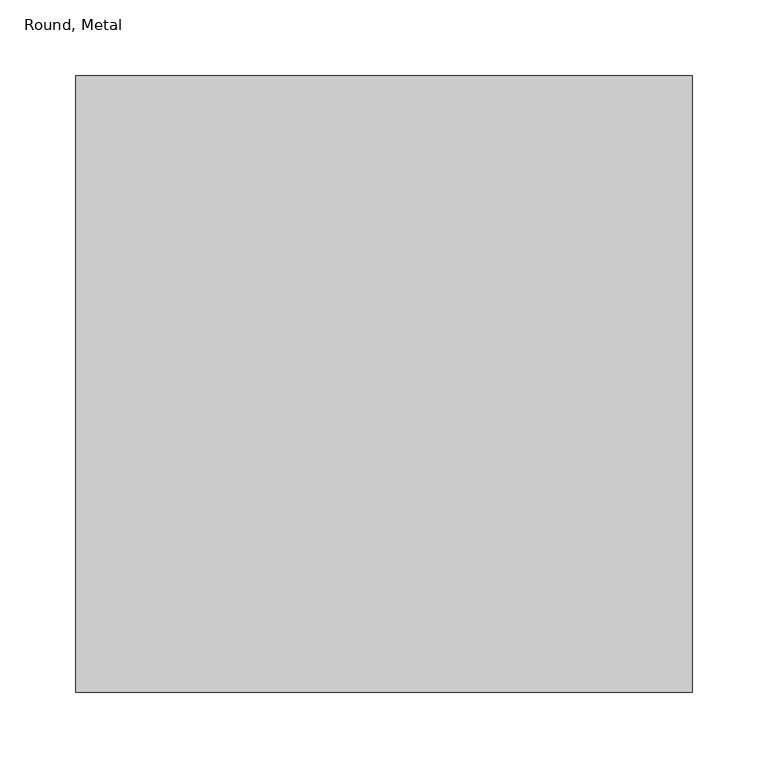
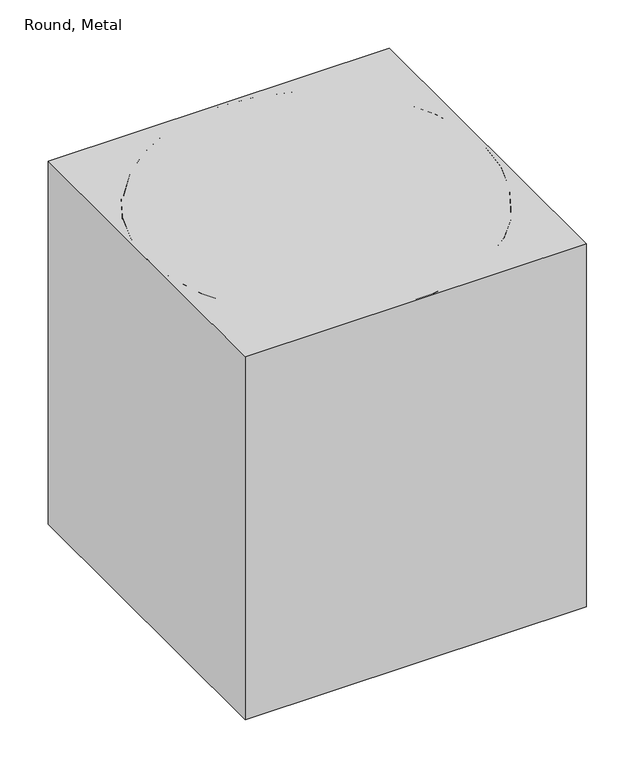
"""IFC4 building model written with IfcOpenShell, lengths in millimetres: proxy geometry, F2000 - Basket, Wastepaper : Round, Metal."""

import ifcopenshell
import ifcopenshell.guid

model = None  # the IFC model being written
_history = None  # IfcOwnerHistory: only IFC2X3 demands one
_inside = {}  # id of a spatial element -> (the spatial element, [elements in it])
_under = {}  # id of a project, library or spatial element -> (it, [spatial elements below it])
_declared = {}  # id of a project -> (the project, [libraries it declares])
_typed = {}  # id of a type object -> (the type object, [elements of that type])
_made_of = {}  # id of a material, layer set ... -> (it, [elements and type objects made of it])


def new_model(schema):
    """Start an empty IFC model of exactly this schema.

    Asked for "IFC4X3", IfcOpenShell would pick the latest addendum, in which some entities
    have other attributes; the version numbers below select the first issue.
    IFC2X3 requires an IfcOwnerHistory on every rooted entity: one is made here for all.
    """
    global model, _history
    if schema == "IFC4X3":
        model = ifcopenshell.file(schema_version=(4, 3, 0, 0))
    else:
        model = ifcopenshell.file(schema=schema)
    _inside.clear()
    _under.clear()
    _declared.clear()
    _typed.clear()
    _made_of.clear()
    _history = None
    if model.schema == "IFC2X3":
        org = make("IfcOrganization", Name="unknown")
        user = make(
            "IfcPersonAndOrganization",
            ThePerson=make("IfcPerson", FamilyName="unknown"),
            TheOrganization=org,
        )
        app = make(
            "IfcApplication",
            ApplicationDeveloper=org,
            Version="unknown",
            ApplicationFullName="unknown",
            ApplicationIdentifier="unknown",
        )
        _history = make(
            "IfcOwnerHistory",
            OwningUser=user,
            OwningApplication=app,
            ChangeAction="ADDED",
            CreationDate=0,
        )
    return model


def make(cls, **values):
    """One entity of the class cls with the attributes given. An attribute that is None is left unset."""
    return model.create_entity(
        cls, **{name: value for name, value in values.items() if value is not None}
    )


def rooted(cls, **values):
    """An entity with a GlobalId (a new one), such as an element, a storey or a relation."""
    return make(cls, GlobalId=ifcopenshell.guid.new(), OwnerHistory=_history, **values)


def si_unit(unit_type, name, prefix=None):
    """IfcSIUnit, for example si_unit("LENGTHUNIT", "METRE", prefix="MILLI")."""
    return make("IfcSIUnit", UnitType=unit_type, Prefix=prefix, Name=name)


def assignment(units):
    """IfcUnitAssignment: the units of a project."""
    return None if units is None else make("IfcUnitAssignment", Units=units)


def point(xyz):
    """IfcCartesianPoint."""
    return None if xyz is None else make("IfcCartesianPoint", Coordinates=xyz)


def direction(xyz):
    """IfcDirection."""
    return None if xyz is None else make("IfcDirection", DirectionRatios=xyz)


def frame(location, z_axis=None, x_axis=None):
    """IfcAxis2Placement3D, a coordinate frame: its origin and axes. An axis left out is left unset."""
    return make(
        "IfcAxis2Placement3D",
        Location=point(location),
        Axis=direction(z_axis),
        RefDirection=direction(x_axis),
    )


def frame_2d(location, x_axis=None):
    """IfcAxis2Placement2D, a coordinate frame in the plane: its origin and x axis."""
    return make(
        "IfcAxis2Placement2D", Location=point(location), RefDirection=direction(x_axis)
    )


def origin():
    """The frame at (0, 0, 0) with its axes left unset."""
    return frame((0.0, 0.0, 0.0))


def origin_with_axes():
    """The frame at (0, 0, 0) with the z axis (0, 0, 1) and the x axis (1, 0, 0) written out."""
    return frame((0.0, 0.0, 0.0), z_axis=(0.0, 0.0, 1.0), x_axis=(1.0, 0.0, 0.0))


def origin_2d():
    """The frame at (0, 0) in the plane with its x axis left unset."""
    return frame_2d((0.0, 0.0))


def place(relative_to, where):
    """IfcLocalPlacement: puts the frame where relative to a parent placement (None: the world)."""
    return make(
        "IfcLocalPlacement", PlacementRelTo=relative_to, RelativePlacement=where
    )


def context(
    kind, dimensions, precision=None, world=None, true_north=None, identifier=None
):
    """IfcGeometricRepresentationContext, for example the 3D "Model" context."""
    return make(
        "IfcGeometricRepresentationContext",
        ContextIdentifier=identifier,
        ContextType=kind,
        CoordinateSpaceDimension=dimensions,
        Precision=precision,
        WorldCoordinateSystem=world,
        TrueNorth=true_north,
    )


def project(units=None, contexts=None):
    """IfcProject with its units and contexts."""
    return rooted(
        "IfcProject",
        Name="project",
        RepresentationContexts=contexts,
        UnitsInContext=assignment(units),
    )


def spatial(cls, under=None, at=None, **own):
    """A site, building, storey or space (cls), placed at a placement, below another one or the project."""
    s = rooted(cls, ObjectPlacement=at, **own)
    if under is not None:
        _under.setdefault(under.id(), (under, []))[1].append(s)
    return s


def polyline(points):
    """IfcPolyline through the points."""
    return make("IfcPolyline", Points=[point(p) for p in points])


def circle_curve(where, radius):
    """IfcCircle in the frame where."""
    return make("IfcCircle", Position=where, Radius=radius)


def trimmed(basis, trim1, trim2, sense, master):
    """IfcTrimmedCurve: the piece of a basis curve between two trims."""
    return make(
        "IfcTrimmedCurve",
        BasisCurve=basis,
        Trim1=trim1,
        Trim2=trim2,
        SenseAgreement=sense,
        MasterRepresentation=master,
    )


def segment(curve, same_sense, transition):
    """IfcCompositeCurveSegment."""
    return make(
        "IfcCompositeCurveSegment",
        Transition=transition,
        SameSense=same_sense,
        ParentCurve=curve,
    )


def composite_curve(segments, self_intersect=None):
    """IfcCompositeCurve: segments joined end to end."""
    return make("IfcCompositeCurve", Segments=segments, SelfIntersect=self_intersect)


def outline(outer, holes=None, kind="AREA"):
    """IfcArbitraryClosedProfileDef: a profile drawn as a closed curve; with holes, ...WithVoids."""
    if holes is None:
        return make("IfcArbitraryClosedProfileDef", ProfileType=kind, OuterCurve=outer)
    return make(
        "IfcArbitraryProfileDefWithVoids",
        ProfileType=kind,
        OuterCurve=outer,
        InnerCurves=holes,
    )


def extrude(swept, where, along, depth):
    """IfcExtrudedAreaSolid: the profile swept, set in the frame where, extruded along a direction by depth."""
    return make(
        "IfcExtrudedAreaSolid",
        SweptArea=swept,
        Position=where,
        ExtrudedDirection=direction(along),
        Depth=depth,
    )


def shape(context_of_items, identifier, shape_type, items):
    """IfcShapeRepresentation: the items that make up one representation, for example the "Body"."""
    return make(
        "IfcShapeRepresentation",
        ContextOfItems=context_of_items,
        RepresentationIdentifier=identifier,
        RepresentationType=shape_type,
        Items=items,
    )


def source(mapping_origin, context_of_items, identifier, shape_type, items):
    """IfcRepresentationMap: a shape defined once, which mapped items show again and again."""
    return make(
        "IfcRepresentationMap",
        MappingOrigin=mapping_origin,
        MappedRepresentation=shape(context_of_items, identifier, shape_type, items),
    )


def transform(
    local_origin,
    x_axis=None,
    y_axis=None,
    z_axis=None,
    scale=None,
    scale2=None,
    scale3=None,
    uniform=True,
):
    """IfcCartesianTransformationOperator3D, or its non-uniform kind. x_axis, y_axis, z_axis: its Axis1, 2, 3."""
    if uniform:
        return make(
            "IfcCartesianTransformationOperator3D",
            Axis1=direction(x_axis),
            Axis2=direction(y_axis),
            LocalOrigin=point(local_origin),
            Scale=scale,
            Axis3=direction(z_axis),
        )
    return make(
        "IfcCartesianTransformationOperator3DnonUniform",
        Axis1=direction(x_axis),
        Axis2=direction(y_axis),
        LocalOrigin=point(local_origin),
        Scale=scale,
        Axis3=direction(z_axis),
        Scale2=scale2,
        Scale3=scale3,
    )


def mapped(mapping_source, mapping_target):
    """IfcMappedItem: shows the shape of a source again, moved by a transform."""
    return make(
        "IfcMappedItem", MappingSource=mapping_source, MappingTarget=mapping_target
    )


def made_of(thing, what):
    """Note that an element or type object is made of a material, layer set ...; save() writes the relation."""
    if what is not None:
        _made_of.setdefault(what.id(), (what, []))[1].append(thing)
    return thing


def element(
    cls,
    number,
    at=None,
    inside=None,
    cuts=None,
    type_object=None,
    material=None,
    context=None,
    identifier="Body",
    shape_type=None,
    held_by="IfcProductDefinitionShape",
    body=None,
    shapes=None,
    **own,
):
    """One element of the class cls, such as IfcWall. Its Tag is "e" and its number.

    at: its placement. inside: the storey or other place that contains it. cuts: it is an
    opening in that element (IfcRelVoidsElement). A single representation is given by context,
    identifier, shape_type and body (its items); several are given by shapes. held_by: the class
    of the entity that holds the representations. save() writes the other relations.
    """
    e = rooted(cls, Tag="e%d" % number, ObjectPlacement=at, **own)
    if body is not None:
        shapes = [shape(context, identifier, shape_type, body)]
    if shapes is not None:
        e.Representation = make(held_by, Representations=shapes)
    if inside is not None:
        _inside.setdefault(inside.id(), (inside, []))[1].append(e)
    if cuts is not None:
        rooted(
            "IfcRelVoidsElement", RelatingBuildingElement=cuts, RelatedOpeningElement=e
        )
    if type_object is not None:
        _typed.setdefault(type_object.id(), (type_object, []))[1].append(e)
    return made_of(e, material)


def aggregate(whole, parts):
    """IfcRelAggregates: a whole, such as a stair, and the parts it consists of."""
    return rooted("IfcRelAggregates", RelatingObject=whole, RelatedObjects=parts)


def save(model, path):
    """Write the relations noted so far, then the file.

    IfcRelAggregates (storeys below a building ...), IfcRelContainedInSpatialStructure (elements
    in a storey), IfcRelDefinesByType, IfcRelAssociatesMaterial and IfcRelDeclares: one each for
    every whole, place, type object, material and project.
    """
    for whole, parts in _under.values():
        aggregate(whole, parts)
    for where, things in _inside.values():
        rooted(
            "IfcRelContainedInSpatialStructure",
            RelatedElements=things,
            RelatingStructure=where,
        )
    for kind, things in _typed.values():
        rooted("IfcRelDefinesByType", RelatedObjects=things, RelatingType=kind)
    for what, things in _made_of.values():
        rooted("IfcRelAssociatesMaterial", RelatedObjects=things, RelatingMaterial=what)
    for by, libraries in _declared.values():
        rooted("IfcRelDeclares", RelatingContext=by, RelatedDefinitions=libraries)
    model.write(path)


def round_metal_5d4f5fea(model_context):
    return source(origin(), model_context, "Body", "SweptSolid", [
        extrude(outline(polyline([(203.2, 203.2), (203.2, -203.2), (-203.2, -203.2), (-203.2, 203.2), (203.2, 203.2)])), origin_with_axes(), (0.0, 0.0, 1.0), 457.2),
        extrude(outline(composite_curve([segment(trimmed(circle_curve(origin_2d(), 203.2), [point((-203.2, 0.0))], [point((203.2, 0.0))], False, "CARTESIAN"), True, "CONTINUOUS"), segment(trimmed(circle_curve(origin_2d(), 203.2), [point((203.2, 0.0))], [point((-203.2, 0.0))], False, "CARTESIAN"), True, "CONTINUOUS")], self_intersect=False)), origin_with_axes(), (0.0, 0.0, 1.0), 3.175),
        extrude(outline(composite_curve([segment(trimmed(circle_curve(origin_2d(), 203.2), [point((-203.2, 0.0))], [point((203.2, 0.0))], False, "CARTESIAN"), True, "CONTINUOUS"), segment(trimmed(circle_curve(origin_2d(), 203.2), [point((203.2, 0.0))], [point((-203.2, 0.0))], False, "CARTESIAN"), True, "CONTINUOUS")], self_intersect=False), holes=[composite_curve([segment(trimmed(circle_curve(origin_2d(), 200.025), [point((-200.025, 0.0))], [point((200.025, 0.0))], True, "CARTESIAN"), True, "CONTINUOUS"), segment(trimmed(circle_curve(origin_2d(), 200.025), [point((200.025, 0.0))], [point((-200.025, 0.0))], True, "CARTESIAN"), True, "CONTINUOUS")], self_intersect=False)]), frame((0.0, 0.0, 3.175), z_axis=(0.0, 0.0, 1.0), x_axis=(1.0, 0.0, 0.0)), (0.0, 0.0, 1.0), 454.025),
    ])


if __name__ == "__main__":
    model = new_model("IFC4")
    model_context = context("Model", 3, world=origin())
    ifc_project = project(units=[si_unit("LENGTHUNIT", "METRE", prefix="MILLI")], contexts=[model_context])
    site = spatial("IfcSite", under=ifc_project)
    building = spatial("IfcBuilding", under=site)
    placement = place(None, origin())
    round_metal_shape = round_metal_5d4f5fea(model_context)
    element("IfcBuildingElementProxy", 1, Name="F2000 - Basket, Wastepaper : Round, Metal", ObjectType="F2000 - Basket, Wastepaper : Round, Metal", at=placement, inside=building, context=model_context, shape_type="MappedRepresentation", body=[
        mapped(round_metal_shape, transform((0.0, 0.0, 0.0), x_axis=(1.0, 0.0, 0.0), y_axis=(0.0, 1.0, 0.0), z_axis=(0.0, 0.0, 1.0))),
    ])
    save(model, "model.ifc")

# Revit data of these elements
# Project information
#   Room Abbreviation = "XVC01"
#   Room Description = "X-Ray, Viewing/Consultation (XVC01)"
#   Sheets - Total = "5"
#   Project Issue Date = "Issue Date"
#   Project Status = "Project Status"
#   Client Name = "Owner"
#   Project Address = "Enter address here"
#   Project Name = "Project Name"
#   Project Number = "Project Number"
#   Publication Date = "1-Feb-16"
# Type "F2000 - Basket, Wastepaper : Round, Metal"
#   Watts2 = "0"
#   Watts1 = "0"
#   Unit_Issue = "EA"
#   UTIL_6_Misc = "-"
#   UTIL_5_NonMedGas = "-"
#   UTIL_4_MiscGas = "-"
#   UTIL_3_MedGas = "-"
#   UTIL_2_Elec = "-"
#   UTIL_1_WaterDrain = "-"
#   Nomenclature = "Basket, Wastepaper, Round, Metal"
#   NSN = "7520002051857"
#   Location [instance default] = ""
#   JSN = "F2000"
#   Fund_Source_VA = "-"
#   Fund_Source_Navy = "-"
#   Fund_Source_Army = "-"
#   Fund_Source_AF = "-"
#   ELEC_Volts2 = "0"
#   ELEC_Volts1 = "0"
#   ELEC_Phase2 = "0"
#   ELEC_Phase1 = "0"
#   ELEC_HertzSwitch = "0"
#   ELEC_HertzDependent = "0"
#   ELEC_Hertz = "0"
#   ELEC_Amps2 = "0"
#   ELEC_Amps1 = "0"
#   DetailDescription = "Round wastepaper basket, approximately 18\" high X 16\" diameter. This metal unit is used to collect and temporarily store small quantities of paper refuse in patient rooms, administrative areas and nursing stations."
#   CAT_VA = "C"
#   CAT_Navy = "C"
#   CAT_IHS = "-"
#   CAT_Army = "C"
#   CAT_AF = "C"
#   BTUperhour = "0"
#   Weight_IP = 6
#   DIM_Width_IP = 1' - 4"
#   DIM_Height_IP = 1' - 6"
#   DIM_Depth_IP = 1' - 4"
#   Assembly Code = ""
# Element 1 (IfcBuildingElementProxy, "F2000 - Basket, Wastepaper : Round, Metal")
#   Location = "XVC01"
#   Materials on its faces: "EquipSpace"
# Materials
#   "EquipSpace": class "Unassigned", colour RGB 221 217 195, transparency 0.5
